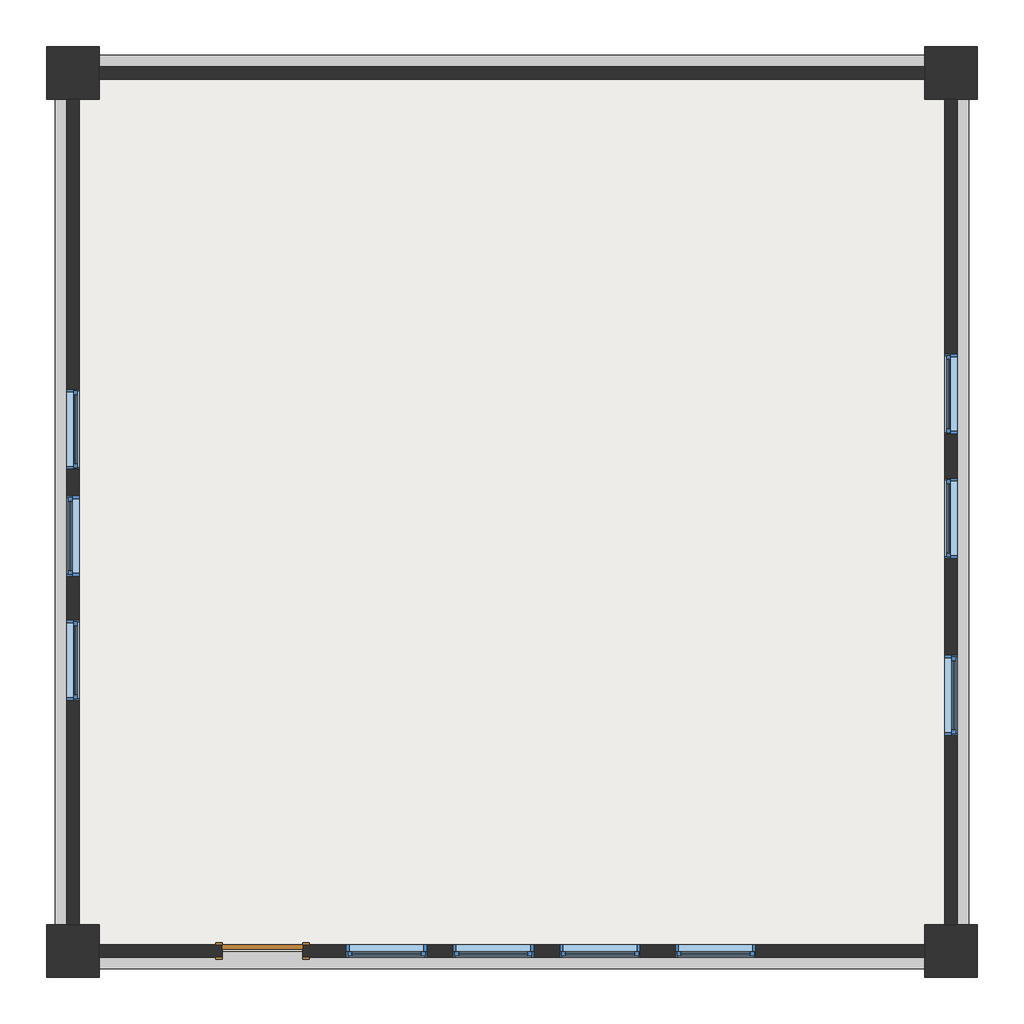
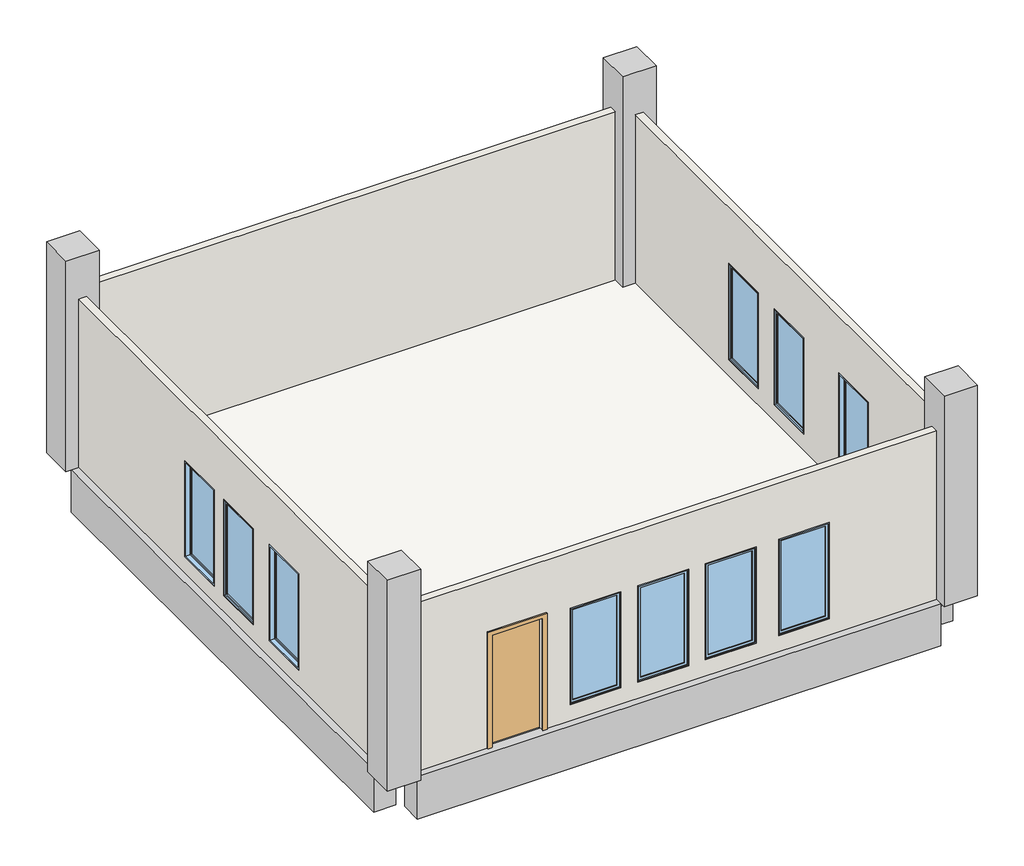
# One storey: 10 windows, 4 beams, 4 columns, 4 walls, 1 door, 1 slab.
"""IFC4 building model written with IfcOpenShell, lengths in millimetres."""

import ifcopenshell
import ifcopenshell.guid

model = None  # the IFC model being written
_history = None  # IfcOwnerHistory: only IFC2X3 demands one
_inside = {}  # id of a spatial element -> (the spatial element, [elements in it])
_under = {}  # id of a project, library or spatial element -> (it, [spatial elements below it])
_declared = {}  # id of a project -> (the project, [libraries it declares])
_typed = {}  # id of a type object -> (the type object, [elements of that type])
_made_of = {}  # id of a material, layer set ... -> (it, [elements and type objects made of it])


def new_model(schema):
    """Start an empty IFC model of exactly this schema.

    Asked for "IFC4X3", IfcOpenShell would pick the latest addendum, in which some entities
    have other attributes; the version numbers below select the first issue.
    IFC2X3 requires an IfcOwnerHistory on every rooted entity: one is made here for all.
    """
    global model, _history
    if schema == "IFC4X3":
        model = ifcopenshell.file(schema_version=(4, 3, 0, 0))
    else:
        model = ifcopenshell.file(schema=schema)
    _inside.clear()
    _under.clear()
    _declared.clear()
    _typed.clear()
    _made_of.clear()
    _history = None
    if model.schema == "IFC2X3":
        org = make("IfcOrganization", Name="unknown")
        user = make(
            "IfcPersonAndOrganization",
            ThePerson=make("IfcPerson", FamilyName="unknown"),
            TheOrganization=org,
        )
        app = make(
            "IfcApplication",
            ApplicationDeveloper=org,
            Version="unknown",
            ApplicationFullName="unknown",
            ApplicationIdentifier="unknown",
        )
        _history = make(
            "IfcOwnerHistory",
            OwningUser=user,
            OwningApplication=app,
            ChangeAction="ADDED",
            CreationDate=0,
        )
    return model


def make(cls, **values):
    """One entity of the class cls with the attributes given. An attribute that is None is left unset."""
    return model.create_entity(
        cls, **{name: value for name, value in values.items() if value is not None}
    )


def rooted(cls, **values):
    """An entity with a GlobalId (a new one), such as an element, a storey or a relation."""
    return make(cls, GlobalId=ifcopenshell.guid.new(), OwnerHistory=_history, **values)


def si_unit(unit_type, name, prefix=None):
    """IfcSIUnit, for example si_unit("LENGTHUNIT", "METRE", prefix="MILLI")."""
    return make("IfcSIUnit", UnitType=unit_type, Prefix=prefix, Name=name)


def assignment(units):
    """IfcUnitAssignment: the units of a project."""
    return None if units is None else make("IfcUnitAssignment", Units=units)


def point(xyz):
    """IfcCartesianPoint."""
    return None if xyz is None else make("IfcCartesianPoint", Coordinates=xyz)


def direction(xyz):
    """IfcDirection."""
    return None if xyz is None else make("IfcDirection", DirectionRatios=xyz)


def frame(location, z_axis=None, x_axis=None):
    """IfcAxis2Placement3D, a coordinate frame: its origin and axes. An axis left out is left unset."""
    return make(
        "IfcAxis2Placement3D",
        Location=point(location),
        Axis=direction(z_axis),
        RefDirection=direction(x_axis),
    )


def origin():
    """The frame at (0, 0, 0) with its axes left unset."""
    return frame((0.0, 0.0, 0.0))


def origin_with_axes():
    """The frame at (0, 0, 0) with the z axis (0, 0, 1) and the x axis (1, 0, 0) written out."""
    return frame((0.0, 0.0, 0.0), z_axis=(0.0, 0.0, 1.0), x_axis=(1.0, 0.0, 0.0))


def place(relative_to, where):
    """IfcLocalPlacement: puts the frame where relative to a parent placement (None: the world)."""
    return make(
        "IfcLocalPlacement", PlacementRelTo=relative_to, RelativePlacement=where
    )


def context(
    kind, dimensions, precision=None, world=None, true_north=None, identifier=None
):
    """IfcGeometricRepresentationContext, for example the 3D "Model" context."""
    return make(
        "IfcGeometricRepresentationContext",
        ContextIdentifier=identifier,
        ContextType=kind,
        CoordinateSpaceDimension=dimensions,
        Precision=precision,
        WorldCoordinateSystem=world,
        TrueNorth=true_north,
    )


def project(units=None, contexts=None):
    """IfcProject with its units and contexts."""
    return rooted(
        "IfcProject",
        Name="project",
        RepresentationContexts=contexts,
        UnitsInContext=assignment(units),
    )


def spatial(cls, under=None, at=None, **own):
    """A site, building, storey or space (cls), placed at a placement, below another one or the project."""
    s = rooted(cls, ObjectPlacement=at, **own)
    if under is not None:
        _under.setdefault(under.id(), (under, []))[1].append(s)
    return s


def polyline(points):
    """IfcPolyline through the points."""
    return make("IfcPolyline", Points=[point(p) for p in points])


def outline(outer, holes=None, kind="AREA"):
    """IfcArbitraryClosedProfileDef: a profile drawn as a closed curve; with holes, ...WithVoids."""
    if holes is None:
        return make("IfcArbitraryClosedProfileDef", ProfileType=kind, OuterCurve=outer)
    return make(
        "IfcArbitraryProfileDefWithVoids",
        ProfileType=kind,
        OuterCurve=outer,
        InnerCurves=holes,
    )


def extrude(swept, where, along, depth):
    """IfcExtrudedAreaSolid: the profile swept, set in the frame where, extruded along a direction by depth."""
    return make(
        "IfcExtrudedAreaSolid",
        SweptArea=swept,
        Position=where,
        ExtrudedDirection=direction(along),
        Depth=depth,
    )


def faces_of(points, faces, orient=None, outer=None):
    """IfcFace entities. A face is a list of loops; a loop is a list of indices into points, from 0.

    orient and outer hold one flag for each loop. By default every Orientation is true, the
    first loop of a face is its IfcFaceOuterBound and the others are IfcFaceBound.
    """
    made = []
    for i, loops in enumerate(faces):
        bounds = []
        for j, loop in enumerate(loops):
            is_outer = j == 0 if outer is None else outer[i][j]
            bounds.append(
                make(
                    "IfcFaceOuterBound" if is_outer else "IfcFaceBound",
                    Bound=make("IfcPolyLoop", Polygon=[points[k] for k in loop]),
                    Orientation=True if orient is None else orient[i][j],
                )
            )
        made.append(make("IfcFace", Bounds=bounds))
    return made


def faceted_brep(points, faces, orient=None, outer=None, voids=None):
    """IfcFacetedBrep: a solid bounded by flat faces; with voids (closed shells), ...WithVoids."""
    shared = [point(p) for p in points]
    hull = make("IfcClosedShell", CfsFaces=faces_of(shared, faces, orient, outer))
    if voids is None:
        return make("IfcFacetedBrep", Outer=hull)
    return make(
        "IfcFacetedBrepWithVoids",
        Outer=hull,
        Voids=[
            make(cls, CfsFaces=faces_of(shared, fs, o, b)) for cls, fs, o, b in voids
        ],
    )


def shape(context_of_items, identifier, shape_type, items):
    """IfcShapeRepresentation: the items that make up one representation, for example the "Body"."""
    return make(
        "IfcShapeRepresentation",
        ContextOfItems=context_of_items,
        RepresentationIdentifier=identifier,
        RepresentationType=shape_type,
        Items=items,
    )


def source(mapping_origin, context_of_items, identifier, shape_type, items):
    """IfcRepresentationMap: a shape defined once, which mapped items show again and again."""
    return make(
        "IfcRepresentationMap",
        MappingOrigin=mapping_origin,
        MappedRepresentation=shape(context_of_items, identifier, shape_type, items),
    )


def transform(
    local_origin,
    x_axis=None,
    y_axis=None,
    z_axis=None,
    scale=None,
    scale2=None,
    scale3=None,
    uniform=True,
):
    """IfcCartesianTransformationOperator3D, or its non-uniform kind. x_axis, y_axis, z_axis: its Axis1, 2, 3."""
    if uniform:
        return make(
            "IfcCartesianTransformationOperator3D",
            Axis1=direction(x_axis),
            Axis2=direction(y_axis),
            LocalOrigin=point(local_origin),
            Scale=scale,
            Axis3=direction(z_axis),
        )
    return make(
        "IfcCartesianTransformationOperator3DnonUniform",
        Axis1=direction(x_axis),
        Axis2=direction(y_axis),
        LocalOrigin=point(local_origin),
        Scale=scale,
        Axis3=direction(z_axis),
        Scale2=scale2,
        Scale3=scale3,
    )


def mapped(mapping_source, mapping_target):
    """IfcMappedItem: shows the shape of a source again, moved by a transform."""
    return make(
        "IfcMappedItem", MappingSource=mapping_source, MappingTarget=mapping_target
    )


def made_of(thing, what):
    """Note that an element or type object is made of a material, layer set ...; save() writes the relation."""
    if what is not None:
        _made_of.setdefault(what.id(), (what, []))[1].append(thing)
    return thing


def element(
    cls,
    number,
    at=None,
    inside=None,
    cuts=None,
    type_object=None,
    material=None,
    context=None,
    identifier="Body",
    shape_type=None,
    held_by="IfcProductDefinitionShape",
    body=None,
    shapes=None,
    **own,
):
    """One element of the class cls, such as IfcWall. Its Tag is "e" and its number.

    at: its placement. inside: the storey or other place that contains it. cuts: it is an
    opening in that element (IfcRelVoidsElement). A single representation is given by context,
    identifier, shape_type and body (its items); several are given by shapes. held_by: the class
    of the entity that holds the representations. save() writes the other relations.
    """
    e = rooted(cls, Tag="e%d" % number, ObjectPlacement=at, **own)
    if body is not None:
        shapes = [shape(context, identifier, shape_type, body)]
    if shapes is not None:
        e.Representation = make(held_by, Representations=shapes)
    if inside is not None:
        _inside.setdefault(inside.id(), (inside, []))[1].append(e)
    if cuts is not None:
        rooted(
            "IfcRelVoidsElement", RelatingBuildingElement=cuts, RelatedOpeningElement=e
        )
    if type_object is not None:
        _typed.setdefault(type_object.id(), (type_object, []))[1].append(e)
    return made_of(e, material)


def aggregate(whole, parts):
    """IfcRelAggregates: a whole, such as a stair, and the parts it consists of."""
    return rooted("IfcRelAggregates", RelatingObject=whole, RelatedObjects=parts)


def save(model, path):
    """Write the relations noted so far, then the file.

    IfcRelAggregates (storeys below a building ...), IfcRelContainedInSpatialStructure (elements
    in a storey), IfcRelDefinesByType, IfcRelAssociatesMaterial and IfcRelDeclares: one each for
    every whole, place, type object, material and project.
    """
    for whole, parts in _under.values():
        aggregate(whole, parts)
    for where, things in _inside.values():
        rooted(
            "IfcRelContainedInSpatialStructure",
            RelatedElements=things,
            RelatingStructure=where,
        )
    for kind, things in _typed.values():
        rooted("IfcRelDefinesByType", RelatedObjects=things, RelatingType=kind)
    for what, things in _made_of.values():
        rooted("IfcRelAssociatesMaterial", RelatedObjects=things, RelatingMaterial=what)
    for by, libraries in _declared.values():
        rooted("IfcRelDeclares", RelatingContext=by, RelatedDefinitions=libraries)
    model.write(path)


def door_0915_x_2134mm_8e7afd8c(model_context):
    return source(origin(), model_context, "Body", "SweptSolid", [
        extrude(outline(polyline([(2210.0, -533.5), (0.0, -533.5), (0.0, -457.5), (2134.0, -457.5), (2134.0, 457.5), (0.0, 457.5), (0.0, 533.5), (2210.0, 533.5), (2210.0, -533.5)])), frame((0.0, 70.0, 0.0), z_axis=(0.0, 1.0, 0.0), x_axis=(0.0, 0.0, 1.0)), (0.0, 0.0, 1.0), 25.0),
        extrude(outline(polyline([(2210.0, 533.5), (2210.0, -533.5), (0.0, -533.5), (0.0, -457.5), (2134.0, -457.5), (2134.0, 457.5), (0.0, 457.5), (0.0, 533.5), (2210.0, 533.5)])), frame((0.0, -95.0, 0.0), z_axis=(0.0, 1.0, 0.0), x_axis=(0.0, 0.0, 1.0)), (0.0, 0.0, 1.0), 25.0),
        extrude(outline(polyline([(457.5, 19.0), (-457.5, 19.0), (-457.5, 70.0), (457.5, 70.0), (457.5, 19.0)])), origin_with_axes(), (0.0, 0.0, 1.0), 2134.0),
    ])


def m_fixo_0915_x_1830mm_1cb826ad(model_context):
    return source(origin(), model_context, "Body", "SweptSolid", [
        extrude(outline(polyline([(-394.5, 48.0), (394.5, 48.0), (394.5, 36.0), (-394.5, 36.0), (-394.5, 48.0)])), frame((0.0, 0.0, 368.0), z_axis=(0.0, 0.0, 1.0), x_axis=(1.0, 0.0, 0.0)), (0.0, 0.0, 1.0), 1704.0),
        extrude(outline(polyline([(2116.0, -438.5), (324.0, -438.5), (324.0, 438.5), (2116.0, 438.5), (2116.0, -438.5)]), holes=[polyline([(2072.0, -394.5), (2072.0, 394.5), (368.0, 394.5), (368.0, -394.5), (2072.0, -394.5)])]), frame((0.0, 20.0, 0.0), z_axis=(0.0, 1.0, 0.0), x_axis=(0.0, 0.0, 1.0)), (0.0, 0.0, 1.0), 44.0),
        extrude(outline(polyline([(2135.0, -457.5), (305.0, -457.5), (305.0, 457.5), (2135.0, 457.5), (2135.0, -457.5)]), holes=[polyline([(2116.0, -438.5), (2116.0, 438.5), (324.0, 438.5), (324.0, -438.5), (2116.0, -438.5)])]), frame((0.0, 20.0, 0.0), z_axis=(0.0, 1.0, 0.0), x_axis=(0.0, 0.0, 1.0)), (0.0, 0.0, 1.0), 63.0),
        extrude(outline(polyline([(2135.0, -457.5), (305.0, -457.5), (305.0, 457.5), (2135.0, 457.5), (2135.0, -457.5)]), holes=[polyline([(2103.0, -425.5), (2103.0, 425.5), (337.0, 425.5), (337.0, -425.5), (2103.0, -425.5)])]), frame((0.0, -57.0, 0.0), z_axis=(0.0, 1.0, 0.0), x_axis=(0.0, 0.0, 1.0)), (0.0, 0.0, 1.0), 77.0),
    ])


model = new_model("IFC4")

# Units and contexts
model_context = context("Model", 3, world=origin())
ifc_project = project(units=[si_unit("LENGTHUNIT", "METRE", prefix="MILLI")], contexts=[model_context])

# Site, building, storey
site = spatial("IfcSite", under=ifc_project)
building = spatial("IfcBuilding", under=site)
storey = spatial("IfcBuildingStorey", under=building, Name="Nível 1", Elevation=0.0)

# Beams
placement = place(None, origin())
element("IfcBeam", 1, ObjectType="Concreto-Viga retangular : 400 x 800mm", at=placement, inside=storey, context=model_context, shape_type="SweptSolid", body=[
    extrude(outline(polyline([(6411.329614, -800.0), (6011.329614, -800.0), (6011.329614, -210.0), (6211.329614, -210.0), (6211.329614, 0.0), (6411.329614, 0.0), (6411.329614, -800.0)])), frame((-2623.6821965, 0.0, 0.0), z_axis=(1.0, 0.0, 0.0), x_axis=(0.0, 1.0, 0.0)), (0.0, 0.0, 1.0), 9400.0),
])
element("IfcBeam", 2, ObjectType="Concreto-Viga retangular : 400 x 800mm", at=placement, inside=storey, context=model_context, shape_type="SweptSolid", body=[
    extrude(outline(polyline([(-800.0, 6876.3178035), (-800.0, 7276.3178035), (0.0, 7276.3178035), (0.0, 7076.3178035), (-210.0, 7076.3178035), (-210.0, 6876.3178035), (-800.0, 6876.3178035)])), frame((0.0, -3488.670386, 0.0), z_axis=(0.0, 1.0, 0.0), x_axis=(0.0, 0.0, 1.0)), (0.0, 0.0, 1.0), 9400.0),
])
element("IfcBeam", 3, ObjectType="Concreto-Viga retangular : 400 x 800mm", at=placement, inside=storey, context=model_context, shape_type="SweptSolid", body=[
    extrude(outline(polyline([(-3588.670386, -800.0), (-3988.670386, -800.0), (-3988.670386, 0.0), (-3788.670386, 0.0), (-3788.670386, -210.0), (-3588.670386, -210.0), (-3588.670386, -800.0)])), frame((-2623.6821965, 0.0, 0.0), z_axis=(1.0, 0.0, 0.0), x_axis=(0.0, 1.0, 0.0)), (0.0, 0.0, 1.0), 9400.0),
])
element("IfcBeam", 4, ObjectType="Concreto-Viga retangular : 400 x 800mm", at=placement, inside=storey, context=model_context, shape_type="SweptSolid", body=[
    extrude(outline(polyline([(0.0, -2923.6821965), (0.0, -3123.6821965), (-800.0, -3123.6821965), (-800.0, -2723.6821965), (-210.0, -2723.6821965), (-210.0, -2923.6821965), (0.0, -2923.6821965)])), frame((0.0, -3488.670386, 0.0), z_axis=(0.0, 1.0, 0.0), x_axis=(0.0, 0.0, 1.0)), (0.0, 0.0, 1.0), 9400.0),
])

# Columns
element("IfcColumn", 5, ObjectType="Concreto-Quadrado-Coluna : 600 x 600mm", at=placement, inside=storey, context=model_context, shape_type="SweptSolid", body=[
    extrude(outline(polyline([(-2623.6821965, 6511.329614), (-2623.6821965, 5911.329614), (-3223.6821965, 5911.329614), (-3223.6821965, 6511.329614), (-2623.6821965, 6511.329614)])), origin_with_axes(), (0.0, 0.0, 1.0), 4000.0),
])
element("IfcColumn", 6, ObjectType="Concreto-Quadrado-Coluna : 600 x 600mm", at=placement, inside=storey, context=model_context, shape_type="SweptSolid", body=[
    extrude(outline(polyline([(7376.3178035, 6511.329614), (7376.3178035, 5911.329614), (6776.3178035, 5911.329614), (6776.3178035, 6511.329614), (7376.3178035, 6511.329614)])), origin_with_axes(), (0.0, 0.0, 1.0), 4000.0),
])
element("IfcColumn", 7, ObjectType="Concreto-Quadrado-Coluna : 600 x 600mm", at=placement, inside=storey, context=model_context, shape_type="SweptSolid", body=[
    extrude(outline(polyline([(7376.3178035, -3488.670386), (7376.3178035, -4088.670386), (6776.3178035, -4088.670386), (6776.3178035, -3488.670386), (7376.3178035, -3488.670386)])), origin_with_axes(), (0.0, 0.0, 1.0), 4000.0),
])
element("IfcColumn", 8, ObjectType="Concreto-Quadrado-Coluna : 600 x 600mm", at=placement, inside=storey, context=model_context, shape_type="SweptSolid", body=[
    extrude(outline(polyline([(-2623.6821965, -3488.670386), (-2623.6821965, -4088.670386), (-3223.6821965, -4088.670386), (-3223.6821965, -3488.670386), (-2623.6821965, -3488.670386)])), origin_with_axes(), (0.0, 0.0, 1.0), 4000.0),
])

# Door
door_0915_x_2134mm_shape = door_0915_x_2134mm_8e7afd8c(model_context)
element("IfcDoor", 9, ObjectType="M_Folha única : 0915 x 2134mm", at=placement, inside=storey, context=model_context, shape_type="MappedRepresentation", body=[
    mapped(door_0915_x_2134mm_shape, transform((-766.1821965, -3788.670386, 0.0), x_axis=(1.0, 0.0, 0.0), y_axis=(0.0, 1.0, 0.0), z_axis=(0.0, 0.0, 1.0))),
])

# Slab
element("IfcSlab", 10, ObjectType="Concreto de 160 mm com deck de metal de 50 mm", at=placement, inside=storey, context=model_context, shape_type="Brep", body=[
    faceted_brep([(7076.3178035, 6211.329614, -210.0), (7076.3178035, 5911.329614, -210.0), (7076.3178035, -3488.670386, -210.0), (7076.3178035, -3788.670386, -210.0), (6776.3178035, -3788.670386, -210.0), (-2623.6821965, -3788.670386, -210.0), (-2923.6821965, -3788.670386, -210.0), (-2923.6821965, -3488.670386, -210.0), (-2923.6821965, 5911.329614, -210.0), (-2923.6821965, 6211.329614, -210.0), (-2623.6821965, 6211.329614, -210.0), (6776.3178035, 6211.329614, -210.0), (7076.3178035, 6211.329614, 0.0), (6776.3178035, 6211.329614, 0.0), (-2623.6821965, 6211.329614, 0.0), (-2923.6821965, 6211.329614, 0.0), (-2923.6821965, 5911.329614, 0.0), (-2923.6821965, -3488.670386, 0.0), (-2923.6821965, -3788.670386, 0.0), (-2623.6821965, -3788.670386, 0.0), (6776.3178035, -3788.670386, 0.0), (7076.3178035, -3788.670386, 0.0), (7076.3178035, -3488.670386, 0.0), (7076.3178035, 5911.329614, 0.0)], [[[0, 1, 2, 3, 4, 5, 6, 7, 8, 9, 10, 11]], [[12, 13, 14, 15, 16, 17, 18, 19, 20, 21, 22, 23]], [[3, 2, 1, 0, 12, 23, 22, 21]], [[6, 5, 4, 3, 21, 20, 19, 18]], [[9, 8, 7, 6, 18, 17, 16, 15]], [[0, 11, 10, 9, 15, 14, 13, 12]]]),
])

# Walls
element("IfcWall", 11, ObjectType="Genérico - 140 mm Alvenaria", at=placement, inside=storey, context=model_context, shape_type="SweptSolid", body=[
    extrude(outline(polyline([(-3488.670386, 0.0), (-3488.670386, 3200.0), (5911.329614, 3200.0), (5911.329614, 0.0), (-3488.670386, 0.0)]), holes=[polyline([(2611.329614, 305.0), (2611.329614, 2135.0), (1696.329614, 2135.0), (1696.329614, 305.0), (2611.329614, 305.0)]), polyline([(481.329614, 305.0), (1396.329614, 305.0), (1396.329614, 2135.0), (481.329614, 2135.0), (481.329614, 305.0)]), polyline([(-18.670386, 305.0), (-18.670386, 2135.0), (-933.670386, 2135.0), (-933.670386, 305.0), (-18.670386, 305.0)])]), frame((-2993.6821965, 0.0, 0.0), z_axis=(1.0, 0.0, 0.0), x_axis=(0.0, 1.0, 0.0)), (0.0, 0.0, 1.0), 140.0),
])
element("IfcWall", 12, ObjectType="Genérico - 140 mm Alvenaria", at=placement, inside=storey, context=model_context, shape_type="SweptSolid", body=[
    extrude(outline(polyline([(6776.3178035, 6141.329614), (-2623.6821965, 6141.329614), (-2623.6821965, 6281.329614), (6776.3178035, 6281.329614), (6776.3178035, 6141.329614)])), origin_with_axes(), (0.0, 0.0, 1.0), 3200.0),
])
element("IfcWall", 13, ObjectType="Genérico - 140 mm Alvenaria", at=placement, inside=storey, context=model_context, shape_type="SweptSolid", body=[
    extrude(outline(polyline([(5911.329614, 0.0), (-3488.670386, 0.0), (-3488.670386, 3200.0), (5911.329614, 3200.0), (5911.329614, 0.0)]), holes=[polyline([(2096.329614, 305.0), (3011.329614, 305.0), (3011.329614, 2135.0), (2096.329614, 2135.0), (2096.329614, 305.0)]), polyline([(681.329614, 305.0), (1596.329614, 305.0), (1596.329614, 2135.0), (681.329614, 2135.0), (681.329614, 305.0)]), polyline([(-418.670386, 305.0), (-418.670386, 2135.0), (-1333.670386, 2135.0), (-1333.670386, 305.0), (-418.670386, 305.0)])]), frame((7006.3178035, 0.0, 0.0), z_axis=(1.0, 0.0, 0.0), x_axis=(0.0, 1.0, 0.0)), (0.0, 0.0, 1.0), 140.0),
])
element("IfcWall", 14, ObjectType="Genérico - 140 mm Alvenaria", at=placement, inside=storey, context=model_context, shape_type="SweptSolid", body=[
    extrude(outline(polyline([(2134.0, -308.6821965), (0.0, -308.6821965), (0.0, 6776.3178035), (3200.0, 6776.3178035), (3200.0, -2623.6821965), (0.0, -2623.6821965), (0.0, -1223.6821965), (2134.0, -1223.6821965), (2134.0, -308.6821965)]), holes=[polyline([(305.0, 1106.3178035), (305.0, 191.3178035), (2135.0, 191.3178035), (2135.0, 1106.3178035), (305.0, 1106.3178035)]), polyline([(305.0, 2321.3178035), (305.0, 1406.3178035), (2135.0, 1406.3178035), (2135.0, 2321.3178035), (305.0, 2321.3178035)]), polyline([(305.0, 3536.3178035), (305.0, 2621.3178035), (2135.0, 2621.3178035), (2135.0, 3536.3178035), (305.0, 3536.3178035)]), polyline([(305.0, 4851.3178035), (305.0, 3936.3178035), (2135.0, 3936.3178035), (2135.0, 4851.3178035), (305.0, 4851.3178035)])]), frame((0.0, -3858.670386, 0.0), z_axis=(0.0, 1.0, 0.0), x_axis=(0.0, 0.0, 1.0)), (0.0, 0.0, 1.0), 140.0),
])

# Windows
m_fixo_0915_x_1830mm_shape = m_fixo_0915_x_1830mm_1cb826ad(model_context)
element("IfcWindow", 15, ObjectType="M_Fixo : 0915 x 1830mm", at=placement, inside=storey, context=model_context, shape_type="MappedRepresentation", body=[
    mapped(m_fixo_0915_x_1830mm_shape, transform((648.8178035, -3775.670386, 0.0), x_axis=(-1.0, 0.0, 0.0), y_axis=(0.0, -1.0, 0.0), z_axis=(0.0, 0.0, 1.0))),
])
element("IfcWindow", 16, ObjectType="M_Fixo : 0915 x 1830mm", at=placement, inside=storey, context=model_context, shape_type="MappedRepresentation", body=[
    mapped(m_fixo_0915_x_1830mm_shape, transform((1863.8178035, -3775.670386, 0.0), x_axis=(-1.0, 0.0, 0.0), y_axis=(0.0, -1.0, 0.0), z_axis=(0.0, 0.0, 1.0))),
])
element("IfcWindow", 17, ObjectType="M_Fixo : 0915 x 1830mm", at=placement, inside=storey, context=model_context, shape_type="MappedRepresentation", body=[
    mapped(m_fixo_0915_x_1830mm_shape, transform((3078.8178035, -3775.670386, 0.0), x_axis=(-1.0, 0.0, 0.0), y_axis=(0.0, -1.0, 0.0), z_axis=(0.0, 0.0, 1.0))),
])
element("IfcWindow", 18, ObjectType="M_Fixo : 0915 x 1830mm", at=placement, inside=storey, context=model_context, shape_type="MappedRepresentation", body=[
    mapped(m_fixo_0915_x_1830mm_shape, transform((4393.8178035, -3775.670386, 0.0), x_axis=(-1.0, 0.0, 0.0), y_axis=(0.0, -1.0, 0.0), z_axis=(0.0, 0.0, 1.0))),
])
element("IfcWindow", 19, ObjectType="M_Fixo : 0915 x 1830mm", at=placement, inside=storey, context=model_context, shape_type="MappedRepresentation", body=[
    mapped(m_fixo_0915_x_1830mm_shape, transform((-2936.6821965, 2153.829614, 0.0), x_axis=(0.0, -1.0, 0.0), y_axis=(1.0, 0.0, 0.0), z_axis=(0.0, 0.0, 1.0))),
])
element("IfcWindow", 20, ObjectType="M_Fixo : 0915 x 1830mm", at=placement, inside=storey, context=model_context, shape_type="MappedRepresentation", body=[
    mapped(m_fixo_0915_x_1830mm_shape, transform((-2910.6821965, 938.829614, 0.0), x_axis=(0.0, 1.0, 0.0), y_axis=(-1.0, 0.0, 0.0), z_axis=(0.0, 0.0, 1.0))),
])
element("IfcWindow", 21, ObjectType="M_Fixo : 0915 x 1830mm", at=placement, inside=storey, context=model_context, shape_type="MappedRepresentation", body=[
    mapped(m_fixo_0915_x_1830mm_shape, transform((-2936.6821965, -476.170386, 0.0), x_axis=(0.0, -1.0, 0.0), y_axis=(1.0, 0.0, 0.0), z_axis=(0.0, 0.0, 1.0))),
])
element("IfcWindow", 22, ObjectType="M_Fixo : 0915 x 1830mm", at=placement, inside=storey, context=model_context, shape_type="MappedRepresentation", body=[
    mapped(m_fixo_0915_x_1830mm_shape, transform((7089.3178035, 2553.829614, 0.0), x_axis=(0.0, 1.0, 0.0), y_axis=(-1.0, 0.0, 0.0), z_axis=(0.0, 0.0, 1.0))),
])
element("IfcWindow", 23, ObjectType="M_Fixo : 0915 x 1830mm", at=placement, inside=storey, context=model_context, shape_type="MappedRepresentation", body=[
    mapped(m_fixo_0915_x_1830mm_shape, transform((7089.3178035, 1138.829614, 0.0), x_axis=(0.0, 1.0, 0.0), y_axis=(-1.0, 0.0, 0.0), z_axis=(0.0, 0.0, 1.0))),
])
element("IfcWindow", 24, ObjectType="M_Fixo : 0915 x 1830mm", at=placement, inside=storey, context=model_context, shape_type="MappedRepresentation", body=[
    mapped(m_fixo_0915_x_1830mm_shape, transform((7063.3178035, -876.170386, 0.0), x_axis=(0.0, -1.0, 0.0), y_axis=(1.0, 0.0, 0.0), z_axis=(0.0, 0.0, 1.0))),
])

save(model, "model.ifc")

# Revit data of these elements
# Type "Concreto-Viga retangular : 400 x 800mm"
#   Length [instance default] = 1.524 m
#   b = 0.40 m
#   h = 0.80 m
#   Structural Material [instance default] = Concreto, Moldado in loco, cinza
#   Assembly Code = ""
# Type "Concreto-Quadrado-Coluna : 600 x 600mm"
#   b = 0.60 m
#   Structural Material [instance default] = Concreto, Moldado in loco, cinza
# Type "M_Folha única : 0915 x 2134mm"
#   Type Mark = "20"
#   Construction Type Id = "MDOOR"
#   Analytic Construction = "Metal"
#   Thickness = 0.051 m
#   Thermal Resistance (R) = 0.270117 (m²·K)/W
#   Heat Transfer Coefficient (U) = 3.7021 W/(m²·K)
#   Height = 2.134 m
#   Projeção da apara externa = 0.025 m
#   Projeção da apara interna = 0.025 m
#   Largura da apara = 0.076 m
#   Width = 0.915 m
#   Define Thermal Properties by = 1
#   Define Thermal Properties by = 1
#   Material da porta = Porta - Painel
#   Material da moldura = Porta - Batente
#   Visual Light Transmittance = 0
#   Solar Heat Gain Coefficient = 0
#   Function = (empty or 0)
#   Wall Closure = (empty or 0)
# Type "Concreto de 160 mm com deck de metal de 50 mm"
#   Function = 0
#   Layers, outside or top first: 0.21 m "Concreto, Moldado in loco" (function 1); 0.00 m "Deck de metal" (function 200)
# Type "Genérico - 140 mm Alvenaria"
#   Layers, outside or top first: 0.14 m "Unidades de alvenaria de concreto" (function 1)
# Type "M_Fixo : 0915 x 1830mm"
#   Type Mark = "18"
#   Construction Type Id = "GSP4R"
#   Analytic Construction = "Vidraça única Pilkington 1/8 pol"
#   Visual Light Transmittance = 0.9
#   Thermal Resistance (R) = 0.271106 (m²·K)/W
#   Solar Heat Gain Coefficient = 0.78
#   Heat Transfer Coefficient (U) = 3.6886 W/(m²·K)
#   Height = 1.83 m
#   Altura-padrão do peitoril = 0.305 m
#   Width = 0.915 m
#   Janela aplicada = 0.019 m
#   Define Thermal Properties by = 1
#   Define Thermal Properties by = 1
#   Material da estrutura externa = Caixilho
#   Material da estrutura interna = Caixilho
#   Material do painel de vidro = Vidro
#   Caixilho = Caixilho
#   Wall Closure = (empty or 0)
# Elements 1, 2, 3, 4 (IfcBeam, "Concreto-Viga retangular : 400 x 800mm")
#   Structural Material = Concreto, Moldado in loco, cinza
#   Phase Created = Construção nova
#   Materials on its faces: "Concreto, Moldado in loco, cinza"
# Elements 5, 6, 7, 8 (IfcColumn, "Concreto-Quadrado-Coluna : 600 x 600mm")
#   Structural Material = Concreto, Moldado in loco, cinza
#   Phase Created = Construção nova
#   Materials on its faces: "Concreto, Moldado in loco, cinza"
# Element 9 (IfcDoor, "M_Folha única : 0915 x 2134mm")
#   Phase Created = Construção nova
#   Materials on its faces: "Porta - Batente", "Porta - Painel"
# Element 10 (IfcSlab, "Concreto de 160 mm com deck de metal de 50 mm")
#   Height Offset From Level = 0.00 m
#   built-in parameter 1001954 = 1
#   Phase Created = Construção nova
#   Materials on its faces: "Deck de metal", "Concreto, Moldado in loco"
# Elements 11, 12, 13, 14 (IfcWall, "Genérico - 140 mm Alvenaria")
#   Top Offset = 0.00 m
#   Base Offset = 0.00 m
#   Unconnected Height = 3.20 m
#   wall height = 3.20 m
#   Phase Created = Construção nova
#   Base Constraint = Nível 1
#   Materials on its faces: "Unidades de alvenaria de concreto"
# Element 15 (IfcWindow, "M_Fixo : 0915 x 1830mm")
#   Mark = "1"
#   Phase Created = Construção nova
#   Materials on its faces: "Caixilho", "Vidro"
# Element 16 (IfcWindow, "M_Fixo : 0915 x 1830mm")
#   Mark = "2"
#   Phase Created = Construção nova
#   Materials on its faces: "Caixilho", "Vidro"
# Element 17 (IfcWindow, "M_Fixo : 0915 x 1830mm")
#   Mark = "3"
#   Phase Created = Construção nova
#   Materials on its faces: "Caixilho", "Vidro"
# Element 18 (IfcWindow, "M_Fixo : 0915 x 1830mm")
#   Mark = "4"
#   Phase Created = Construção nova
#   Materials on its faces: "Caixilho", "Vidro"
# Element 19 (IfcWindow, "M_Fixo : 0915 x 1830mm")
#   Mark = "5"
#   Phase Created = Construção nova
#   Materials on its faces: "Caixilho", "Vidro"
# Element 20 (IfcWindow, "M_Fixo : 0915 x 1830mm")
#   Mark = "6"
#   Phase Created = Construção nova
#   Materials on its faces: "Caixilho", "Vidro"
# Element 21 (IfcWindow, "M_Fixo : 0915 x 1830mm")
#   Mark = "7"
#   Phase Created = Construção nova
#   Materials on its faces: "Caixilho", "Vidro"
# Element 22 (IfcWindow, "M_Fixo : 0915 x 1830mm")
#   Mark = "8"
#   Phase Created = Construção nova
#   Materials on its faces: "Caixilho", "Vidro"
# Element 23 (IfcWindow, "M_Fixo : 0915 x 1830mm")
#   Mark = "9"
#   Phase Created = Construção nova
#   Materials on its faces: "Caixilho", "Vidro"
# Element 24 (IfcWindow, "M_Fixo : 0915 x 1830mm")
#   Mark = "10"
#   Phase Created = Construção nova
#   Materials on its faces: "Caixilho", "Vidro"
# Materials
#   "Concreto, Moldado in loco, cinza": class "Concreto", colour RGB 192 192 192, transparency 0, Description = "Concreto moldado in loco", Cost = 0
#   "Porta - Painel": class "Madeira", colour RGB 210 159 95, transparency 0, Cost = 0
#   "Porta - Batente": class "Diversos", colour RGB 118 70 51, transparency 0, Cost = 0
#   "Concreto, Moldado in loco": class "Concreto", colour RGB 192 192 192, transparency 0, Description = "Material físico", Cost = 0
#   "Deck de metal": class "Metal", colour RGB 247 247 247, transparency 0, Description = "Aço, acabamento na usina", Cost = 0
#   "Unidades de alvenaria de concreto": class "Alvenaria", colour RGB 181 181 181, transparency 0, Description = "Unidades de alvenaria de concreto", Cost = 0
#   "Caixilho": class "Madeira", colour RGB 224 178 126, transparency 0, Cost = 0
#   "Vidro": class "Vidro", colour RGB 0 128 192, transparency 0.9, Description = "Vidro de sílica", Cost = 0
